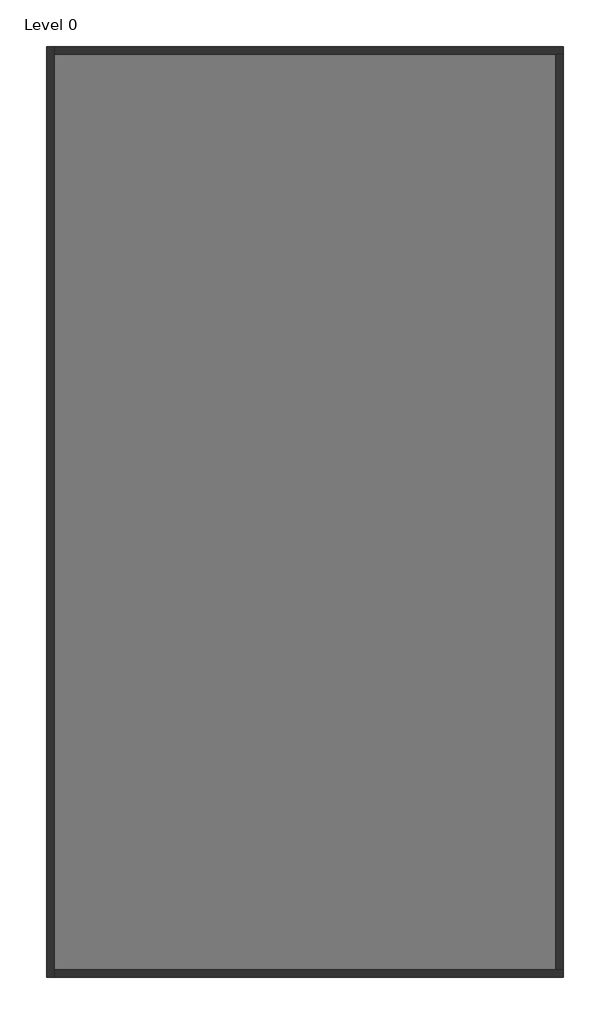
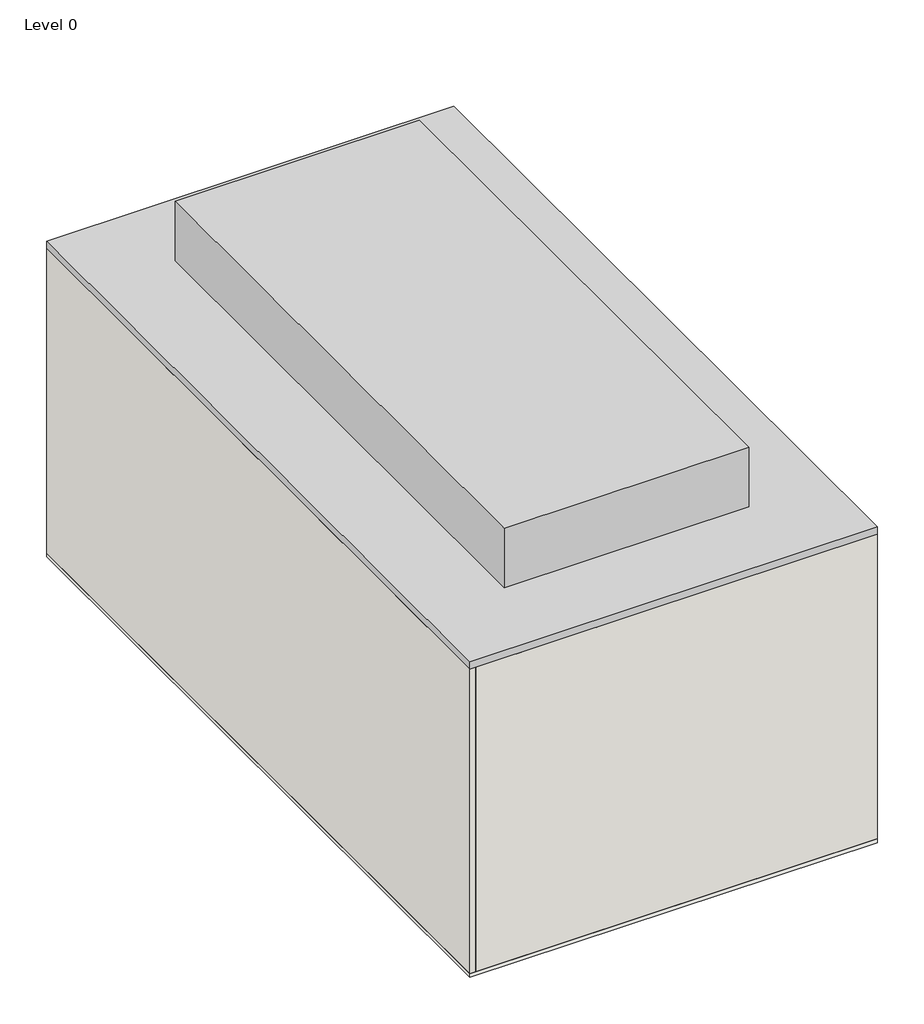
# One storey: 4 walls, 1 proxy, 1 slab.
"""IFC4 building model written with IfcOpenShell, lengths in millimetres."""

from ifc_helpers import new_model, si_unit, frame, origin, origin_with_axes, place, context, project, spatial, polyline, outline, extrude, faceted_brep, element, save

model = new_model("IFC4")

# Units and contexts
model_context = context("Model", 3, world=origin())
ifc_project = project(units=[si_unit("LENGTHUNIT", "METRE", prefix="MILLI")], contexts=[model_context])

# Site, building, storey
site = spatial("IfcSite", under=ifc_project)
building = spatial("IfcBuilding", under=site)
storey = spatial("IfcBuildingStorey", under=building, Name="Level 0", Elevation=100.0)

# Proxy
placement = place(None, origin())
element("IfcBuildingElementProxy", 1, Name="LowUrbanDensityBuilding : LowUrbanDensityBuilding", ObjectType="LowUrbanDensityBuilding : LowUrbanDensityBuilding", at=placement, inside=storey, context=model_context, shape_type="SweptSolid", body=[
    extrude(outline(polyline([(7325.2659446, 3676.2074539), (7325.2659446, -14323.7925461), (-2674.7340554, -14323.7925461), (-2674.7340554, 3676.2074539), (7325.2659446, 3676.2074539)])), origin_with_axes(), (0.0, 0.0, 1.0), 8200.0),
    extrude(outline(polyline([(5325.2659446, 1676.2074539), (5325.2659446, -12323.7925461), (-674.7340554, -12323.7925461), (-674.7340554, 1676.2074539), (5325.2659446, 1676.2074539)])), frame((0.0, 0.0, 8200.0), z_axis=(0.0, 0.0, 1.0), x_axis=(1.0, 0.0, 0.0)), (0.0, 0.0, 1.0), 1549.8),
])

# Slab
element("IfcSlab", 2, ObjectType="Floor-Concrete_100Con", at=placement, inside=storey, context=model_context, shape_type="SweptSolid", body=[
    extrude(outline(polyline([(7325.2659446, 3676.2074539), (7325.2659446, -14323.7925461), (-2674.7340554, -14323.7925461), (-2674.7340554, 3676.2074539), (7325.2659446, 3676.2074539)])), origin_with_axes(), (0.0, 0.0, 1.0), 100.0),
])

# Walls
element("IfcWall", 3, ObjectType="Wall-Ext_25Rdr-100Blk-19P", at=placement, inside=storey, context=model_context, shape_type="Brep", body=[
    faceted_brep([(-2674.7340554, 3676.2074539, 100.0), (-2674.7340554, -14323.7925461, 100.0), (-2674.7340554, -14323.7925461, 8000.0), (-2674.7340554, 3676.2074539, 8000.0), (-2530.4340554, 3676.2074539, 100.0), (-2530.4340554, 3676.2074539, 8000.0), (-2530.4340554, 3531.9074539, 8000.0), (-2530.4340554, -14179.4925461, 8000.0), (-2530.4340554, -14323.7925461, 8000.0), (-2530.4340554, -14323.7925461, 100.0), (-2530.4340554, -14179.4925461, 100.0), (-2530.4340554, 3531.9074539, 100.0)], [[[0, 1, 2, 3]], [[4, 5, 6, 7, 8, 9, 10, 11]], [[1, 0, 4, 11, 10, 9]], [[3, 2, 8, 7, 6, 5]], [[2, 1, 9, 8]], [[0, 3, 5, 4]]]),
])
element("IfcWall", 4, ObjectType="Wall-Ext_25Rdr-100Blk-19P", at=placement, inside=storey, context=model_context, shape_type="Brep", body=[
    faceted_brep([(-2530.4340554, -14323.7925461, 100.0), (7325.2659446, -14323.7925461, 100.0), (7325.2659446, -14323.7925461, 8000.0), (-2530.4340554, -14323.7925461, 8000.0), (-2530.4340554, -14179.4925461, 100.0), (-2530.4340554, -14179.4925461, 8000.0), (7180.9659446, -14179.4925461, 8000.0), (7325.2659446, -14179.4925461, 8000.0), (7325.2659446, -14179.4925461, 100.0), (7180.9659446, -14179.4925461, 100.0)], [[[0, 1, 2, 3]], [[4, 5, 6, 7, 8, 9]], [[1, 0, 4, 9, 8]], [[3, 2, 7, 6, 5]], [[0, 3, 5, 4]], [[2, 1, 8, 7]]]),
])
element("IfcWall", 5, ObjectType="Wall-Ext_25Rdr-100Blk-19P", at=placement, inside=storey, context=model_context, shape_type="Brep", body=[
    faceted_brep([(7325.2659446, 3676.2074539, 100.0), (-2530.4340554, 3676.2074539, 100.0), (-2530.4340554, 3676.2074539, 8000.0), (7325.2659446, 3676.2074539, 8000.0), (7325.2659446, 3531.9074539, 100.0), (7325.2659446, 3531.9074539, 8000.0), (7180.9659446, 3531.9074539, 8000.0), (-2530.4340554, 3531.9074539, 8000.0), (-2530.4340554, 3531.9074539, 100.0), (7180.9659446, 3531.9074539, 100.0)], [[[0, 1, 2, 3]], [[4, 5, 6, 7, 8, 9]], [[1, 0, 4, 9, 8]], [[3, 2, 7, 6, 5]], [[2, 1, 8, 7]], [[0, 3, 5, 4]]]),
])
element("IfcWall", 6, ObjectType="Wall-Ext_25Rdr-100Blk-19P", at=placement, inside=storey, context=model_context, shape_type="SweptSolid", body=[
    extrude(outline(polyline([(7325.2659446, 3531.9074539), (7325.2659446, -14179.4925461), (7180.9659446, -14179.4925461), (7180.9659446, 3531.9074539), (7325.2659446, 3531.9074539)])), frame((0.0, 0.0, 100.0), z_axis=(0.0, 0.0, 1.0), x_axis=(1.0, 0.0, 0.0)), (0.0, 0.0, 1.0), 7900.0),
])

save(model, "model.ifc")

# Revit data of these elements
# Project information
#   Project Issue Date = "Issue Date"
#   Project Status = "Project Status"
#   Client Name = "Owner"
#   Project Address = "Enter address here"
#   Project Name = "Project Name"
#   Project Number = "Project Number"
# Type "Floor-Concrete_100Con"
#   Keynote = "E60/130"
#   Function = 0
#   Layers, outside or top first: 100 mm "Concrete" (function 1)
# Type "Wall-Ext_25Rdr-100Blk-19P"
#   Keynote = "F10"
#   Layers, outside or top first: 25.3 mm "Render, Beige, Smooth" (function 5); 100 mm "Concrete Masonry Units _Low Density" (function 1); 19 mm "Plaster" (function 5)
# Element 1 (IfcBuildingElementProxy, "LowUrbanDensityBuilding : LowUrbanDensityBuilding")
#   Phase Created = New Construction
#   Materials on its faces: "Default Form"
# Element 2 (IfcSlab, "Floor-Concrete_100Con")
#   Height Offset From Level = 0 mm
#   Phase Created = New Construction
#   Materials on its faces: "Concrete"
# Element 3 (IfcWall, "Wall-Ext_25Rdr-100Blk-19P")
#   Top Offset = 0 mm
#   Base Offset = 0 mm
#   wall height = 7900 mm
#   Phase Created = New Construction
#   Base Constraint = Level 0
#   Top Constraint = Level 2
#   Materials on its faces: "Render, Beige, Smooth", "Default Wall", "Plaster"
# Elements 4, 5, 6 (IfcWall, "Wall-Ext_25Rdr-100Blk-19P")
#   Top Offset = 0 mm
#   Base Offset = 0 mm
#   wall height = 7900 mm
#   Phase Created = New Construction
#   Base Constraint = Level 0
#   Top Constraint = Level 2
#   Materials on its faces: "Default Wall", "Render, Beige, Smooth", "Plaster"
# Materials
#   "Concrete": class "Concrete", colour RGB 120 120 120, transparency 0, Description = "Portland Cement Concrete", Cost = 0
#   "Render, Beige, Smooth": class "Generic", colour RGB 213 198 180, transparency 0, Description = "physical material", Cost = 0
#   "Concrete Masonry Units _Low Density": class "Masonry", colour RGB 181 181 181, transparency 0, Description = "Concrete masonry units", Cost = 0
#   "Plaster": class "Generic", colour RGB 249 249 249, transparency 0, Description = "Plaster", Cost = 0
#   "Default Form": class "Generic", colour RGB 185 189 196, transparency 0.5, Cost = 0
#   "Default Wall": class "Miscellaneous", colour RGB 128 128 128, transparency 0, Comments = "Rendering appearance not upgraded Rendering appearance not upgraded ", Cost = 0
